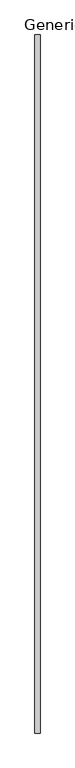
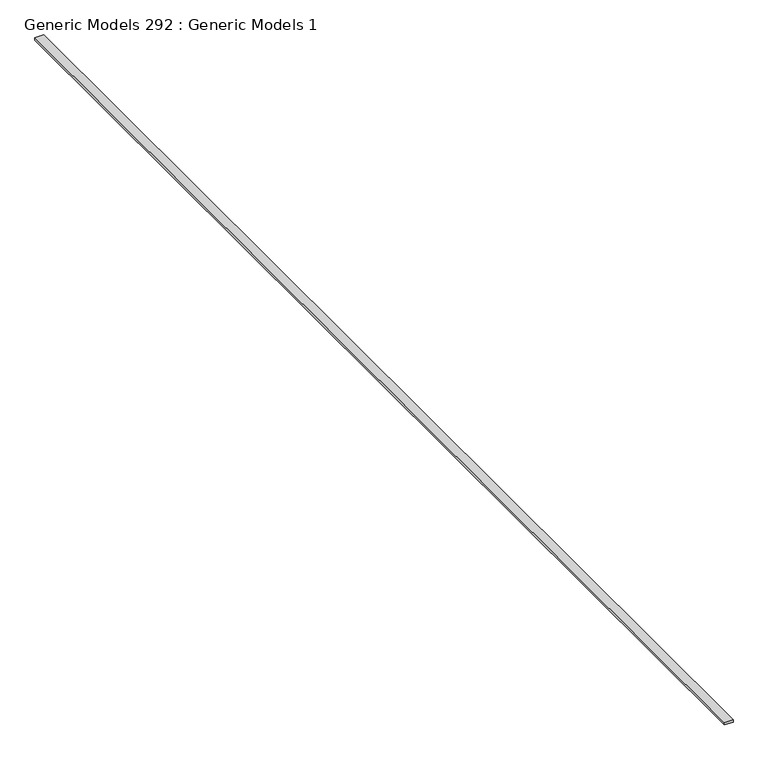
"""IFC4 building model written with IfcOpenShell, lengths in millimetres: proxy geometry, Generic Models 292 : Generic Models 1."""

from ifc_helpers import new_model, si_unit, frame, origin, place, context, project, spatial, polyline, outline, extrude, source, transform, mapped, element, save


def generic_models_292_generic_models_1_5439f6d5(model_context):
    return source(origin(), model_context, "Body", "SweptSolid", [
        extrude(outline(polyline([(26262.2627371, 45695.5591064), (26401.9627371, 45695.5591064), (26401.9627371, 26645.5591064), (26262.2627371, 26645.5591064), (26262.2627371, 45695.5591064)])), frame((0.0, 0.0, 126183.7236113), z_axis=(0.0, 0.0, 1.0), x_axis=(1.0, 0.0, 0.0)), (0.0, 0.0, 1.0), 38.1),
    ])


if __name__ == "__main__":
    model = new_model("IFC4")
    model_context = context("Model", 3, world=origin())
    ifc_project = project(units=[si_unit("LENGTHUNIT", "METRE", prefix="MILLI")], contexts=[model_context])
    site = spatial("IfcSite", under=ifc_project)
    building = spatial("IfcBuilding", under=site)
    placement = place(None, origin())
    generic_models_292_generic_models_1_shape = generic_models_292_generic_models_1_5439f6d5(model_context)
    element("IfcBuildingElementProxy", 1, Name="Generic Models 292 : Generic Models 1", ObjectType="Generic Models 292 : Generic Models 1", at=placement, inside=building, context=model_context, shape_type="MappedRepresentation", body=[
        mapped(generic_models_292_generic_models_1_shape, transform((0.0, 0.0, 0.0), x_axis=(1.0, 0.0, 0.0), y_axis=(0.0, 1.0, 0.0), z_axis=(0.0, 0.0, 1.0))),
    ])
    save(model, "model.ifc")

# Revit data of these elements
# Element 1 (IfcBuildingElementProxy, "Generic Models 292 : Generic Models 1")
#   Materials on its faces: "_2X BLOCKING AS REQUIRED"
# Materials
#   "_2X BLOCKING AS REQUIRED": class "Generic", colour RGB 177 130 114, transparency 0, Cost = 0
